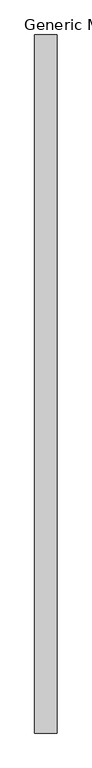
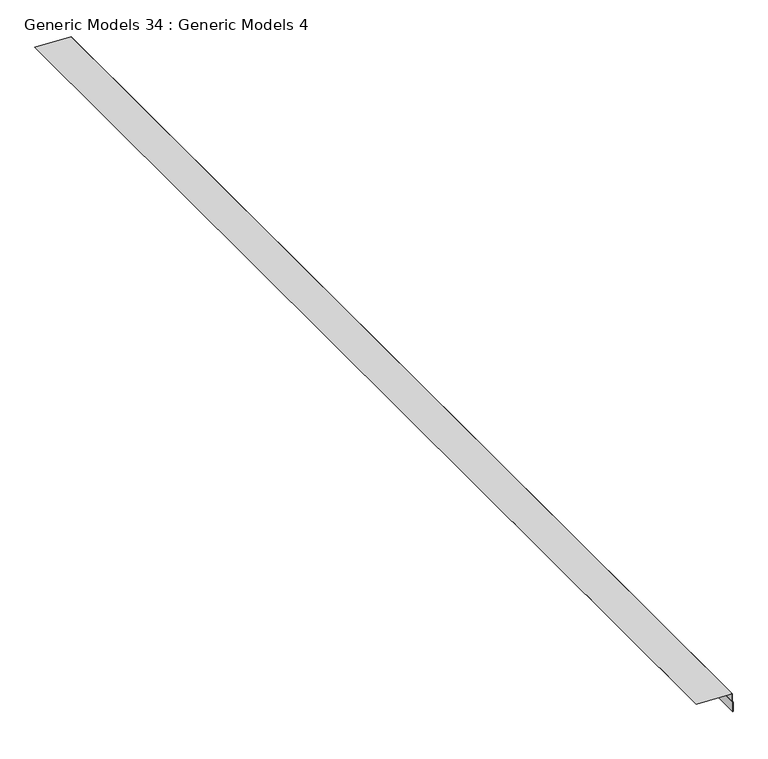
"""IFC4 building model written with IfcOpenShell, lengths in millimetres: proxy geometry, Generic Models 34 : Generic Models 4."""

from ifc_helpers import new_model, si_unit, frame, origin, place, context, project, spatial, polyline, outline, extrude, source, transform, mapped, element, save


def generic_models_34_generic_models_4_204019c3(model_context):
    return source(origin(), model_context, "Body", "SweptSolid", [
        extrude(outline(polyline([(126883.6225001, -9255.4809405), (126841.9533957, -9255.4809405), (126841.9533957, -9254.6871905), (126883.7624596, -9254.6871905), (126890.8944002, -9257.2830045), (126924.5930414, -9257.2830045), (126931.0955684, -9413.3436529), (126930.3025065, -9413.3766972), (126923.8316756, -9258.0767545), (126890.7544406, -9258.0767545), (126883.6225001, -9255.4809405)])), frame((0.0, 7054.2769662, 0.0), z_axis=(0.0, 1.0, 0.0), x_axis=(0.0, 0.0, 1.0)), (0.0, 0.0, 1.0), 4927.6),
    ])


if __name__ == "__main__":
    model = new_model("IFC4")
    model_context = context("Model", 3, world=origin())
    ifc_project = project(units=[si_unit("LENGTHUNIT", "METRE", prefix="MILLI")], contexts=[model_context])
    site = spatial("IfcSite", under=ifc_project)
    building = spatial("IfcBuilding", under=site)
    placement = place(None, origin())
    generic_models_34_generic_models_4_shape = generic_models_34_generic_models_4_204019c3(model_context)
    element("IfcBuildingElementProxy", 1, Name="Generic Models 34 : Generic Models 4", ObjectType="Generic Models 34 : Generic Models 4", at=placement, inside=building, context=model_context, shape_type="MappedRepresentation", body=[
        mapped(generic_models_34_generic_models_4_shape, transform((0.0, 0.0, 0.0), x_axis=(1.0, 0.0, 0.0), y_axis=(0.0, 1.0, 0.0), z_axis=(0.0, 0.0, 1.0))),
    ])
    save(model, "model.ifc")

# Revit data of these elements
# Element 1 (IfcBuildingElementProxy, "Generic Models 34 : Generic Models 4")
#   Materials on its faces: "_(2) LAYERS NO. 30 ASTM D226 ASPHALT SATURATED ORGANIC FELT"
# Materials
#   "_(2) LAYERS NO. 30 ASTM D226 ASPHALT SATURATED ORGANIC FELT": class "Generic", colour RGB 67 154 161, transparency 0, Cost = 0
